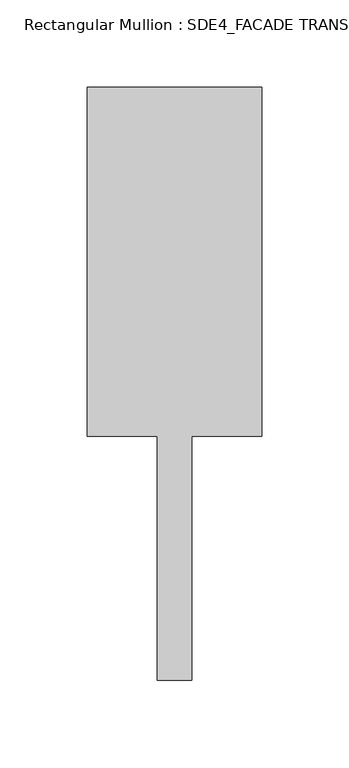
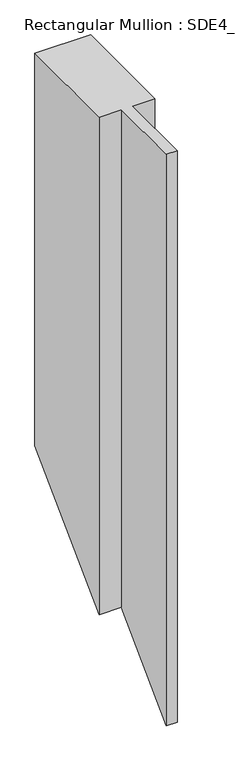
"""IFC4 building model written with IfcOpenShell, lengths in millimetres: member geometry, Rectangular Mullion : SDE4_FACADE TRANSOM TYPE 1."""

from ifc_helpers import new_model, si_unit, origin, place, context, project, spatial, faceted_brep, source, transform, mapped, element, save


def rectangular_mullion_sde4_facade_transom_type_1_bbad81e6(model_context):
    return source(origin(), model_context, "Body", "Brep", [
        faceted_brep([(50.0, 132.5, 0.0), (-50.0, 132.5, 0.0), (-50.0, -67.5, 0.0), (-10.0, -67.5, 0.0), (-10.0, -207.5, 0.0), (10.0, -207.5, 0.0), (10.0, -67.5, 0.0), (50.0, -67.5, 0.0), (50.0, 132.5, -746.0000001), (-50.0, 132.5, -746.0000001), (-50.0, -67.5, -946.0000001), (-10.0, -67.5, -946.0000001), (-10.0, -207.5, -1086.0000001), (10.0, -207.5, -1086.0000001), (10.0, -67.5, -946.0000001), (50.0, -67.5, -946.0000001)], [[[0, 1, 2, 3, 4, 5, 6, 7]], [[1, 0, 8, 9]], [[2, 1, 9, 10]], [[3, 2, 10, 11]], [[4, 3, 11, 12]], [[5, 4, 12, 13]], [[6, 5, 13, 14]], [[7, 6, 14, 15]], [[0, 7, 15, 8]], [[8, 15, 14, 13, 12, 11, 10, 9]]]),
    ])


if __name__ == "__main__":
    model = new_model("IFC4")
    model_context = context("Model", 3, world=origin())
    ifc_project = project(units=[si_unit("LENGTHUNIT", "METRE", prefix="MILLI")], contexts=[model_context])
    site = spatial("IfcSite", under=ifc_project)
    building = spatial("IfcBuilding", under=site)
    placement = place(None, origin())
    rectangular_mullion_sde4_facade_transom_type_1_shape = rectangular_mullion_sde4_facade_transom_type_1_bbad81e6(model_context)
    element("IfcMember", 1, ObjectType="Rectangular Mullion : SDE4_FACADE TRANSOM TYPE 1", at=placement, inside=building, context=model_context, shape_type="MappedRepresentation", body=[
        mapped(rectangular_mullion_sde4_facade_transom_type_1_shape, transform((0.0, 0.0, 0.0), x_axis=(1.0, 0.0, 0.0), y_axis=(0.0, 1.0, 0.0), z_axis=(0.0, 0.0, 1.0))),
    ])
    save(model, "model.ifc")

# Revit data of these elements
# Type "Rectangular Mullion : SDE4_FACADE TRANSOM TYPE 1"
#   built-in parameter 1007322 = 1.11549 (stored number, unit not read)
#   built-in parameter 1007321 = 0.164042 (stored number, unit not read)
#   built-in parameter 1007320 = 0.164042 (stored number, unit not read)
